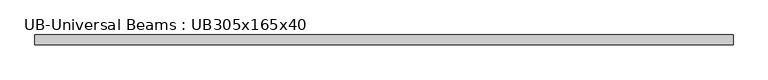
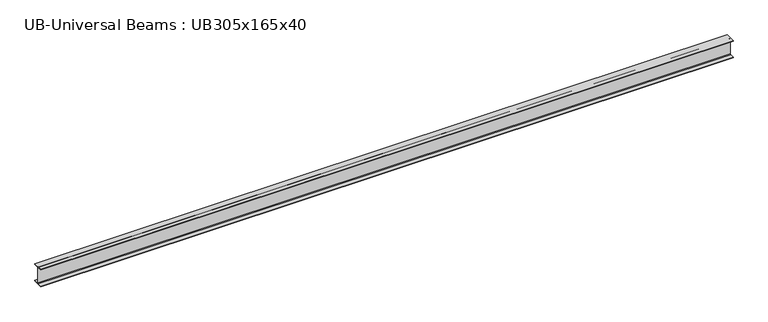
"""IFC4 building model written with IfcOpenShell, lengths in millimetres: member geometry, UB-Universal Beams : UB305x165x40."""

from ifc_helpers import new_model, si_unit, point, frame, frame_2d, origin, place, context, project, spatial, polyline, circle_curve, trimmed, segment, composite_curve, outline, extrude, source, transform, mapped, element, save


def ub_universal_beams_ub305x165x40_27ef7093(model_context):
    return source(origin(), model_context, "Body", "SweptSolid", [
        extrude(outline(composite_curve([segment(polyline([(82.5, -141.5), (82.5, -151.7), (-82.5, -151.7), (-82.5, -141.5), (-11.9, -141.5)]), True, "CONTINUOUS"), segment(trimmed(circle_curve(frame_2d((-11.9, -132.6)), 8.9), [point((-11.9, -141.5))], [point((-3.0, -132.6))], True, "CARTESIAN"), True, "CONTINUOUS"), segment(polyline([(-3.0, -132.6), (-3.0, 132.6)]), True, "CONTINUOUS"), segment(trimmed(circle_curve(frame_2d((-11.9, 132.6)), 8.9), [point((-3.0, 132.6))], [point((-11.9, 141.5))], True, "CARTESIAN"), True, "CONTINUOUS"), segment(polyline([(-11.9, 141.5), (-82.5, 141.5), (-82.5, 151.7), (82.5, 151.7), (82.5, 141.5), (11.9, 141.5)]), True, "CONTINUOUS"), segment(trimmed(circle_curve(frame_2d((11.9, 132.6)), 8.9), [point((11.9, 141.5))], [point((3.0, 132.6))], True, "CARTESIAN"), True, "CONTINUOUS"), segment(polyline([(3.0, 132.6), (3.0, -132.6)]), True, "CONTINUOUS"), segment(trimmed(circle_curve(frame_2d((11.9, -132.6)), 8.9), [point((3.0, -132.6))], [point((11.9, -141.5))], True, "CARTESIAN"), True, "CONTINUOUS"), segment(polyline([(11.9, -141.5), (82.5, -141.5)]), True, "CONTINUOUS")], self_intersect=False)), frame((-5606.85, 0.0, 0.0), z_axis=(1.0, 0.0, 0.0), x_axis=(0.0, 1.0, 0.0)), (0.0, 0.0, 1.0), 11546.3),
    ])


if __name__ == "__main__":
    model = new_model("IFC4")
    model_context = context("Model", 3, world=origin())
    ifc_project = project(units=[si_unit("LENGTHUNIT", "METRE", prefix="MILLI")], contexts=[model_context])
    site = spatial("IfcSite", under=ifc_project)
    building = spatial("IfcBuilding", under=site)
    placement = place(None, origin())
    ub_universal_beams_ub305x165x40_shape = ub_universal_beams_ub305x165x40_27ef7093(model_context)
    element("IfcMember", 1, ObjectType="UB-Universal Beams : UB305x165x40", at=placement, inside=building, context=model_context, shape_type="MappedRepresentation", body=[
        mapped(ub_universal_beams_ub305x165x40_shape, transform((0.0, 0.0, 0.0), x_axis=(1.0, 0.0, 0.0), y_axis=(0.0, 1.0, 0.0), z_axis=(0.0, 0.0, 1.0))),
    ])
    save(model, "model.ifc")

# Revit data of these elements
# Type "UB-Universal Beams : UB305x165x40"
#   Section Name Key = "UB305X165X40"
#   Width = 16.5 cm
#   Web Thickness = 0.6 cm
#   Web Fillet = 0.89 cm
#   Warping Constant = 164000.0 cm⁶
#   Torsional Moment of Inertia = 14.70 cm⁴
#   Section Area = 51.3 cm²
#   Plastic Modulus weak axis = 142.0 cm³
#   Plastic Modulus strong axis = 623.0 cm³
#   Nominal Weight = 40.2999 kgf/m
#   Moment of Inertia weak axis = 764.00 cm⁴
#   Moment of Inertia strong axis = 8503.00 cm⁴
#   Height = 30.34 cm
#   Flange Thickness = 1.02 cm
#   Elastic Modulus weak axis = 92.6 cm³
#   Elastic Modulus strong axis = 560.0 cm³
#   Centroid Vertical = 15.17 cm
#   Centroid Horizontal = 8.25 cm
#   Bolt Spacing = 9.0 cm
#   Length [instance default] = 1500 mm
#   Structural Material [instance default] = Metal - Steel 43-275
#   Type Comments = ""
#   Assembly Code = ""
# Element 1 (IfcMember, "UB-Universal Beams : UB305x165x40")
#   Materials on its faces: "Metal - Steel 43-275"
# Materials
#   "Metal - Steel 43-275": class "Metal", colour RGB 247 247 247, transparency 0, Cost = 0
